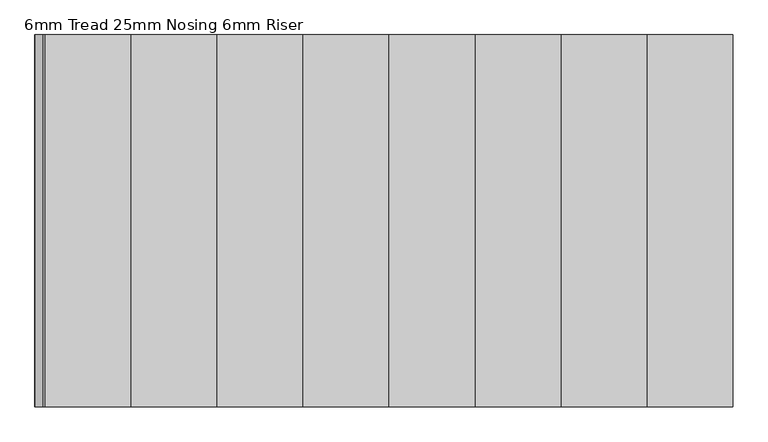
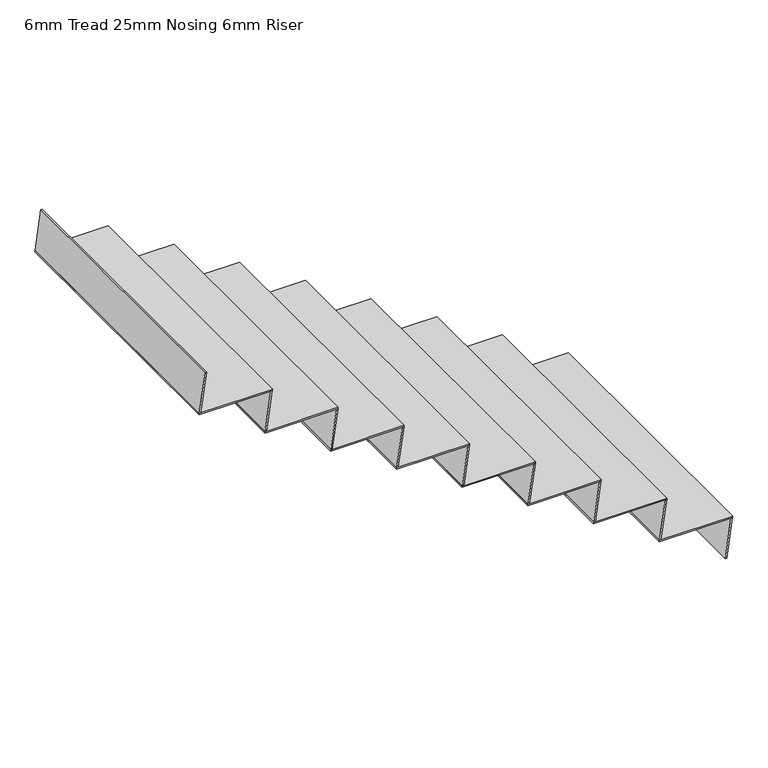
"""IFC4 building model written with IfcOpenShell, lengths in millimetres: stair flight geometry, 6mm Tread 25mm Nosing 6mm Riser."""

from ifc_helpers import new_model, si_unit, frame, origin, place, context, project, spatial, polyline, outline, extrude, source, transform, mapped, element, save


def stair_flight_6mm_tread_25mm_nosing_6mm_riser_aabb701a(model_context):
    return source(origin(), model_context, "Body", "SweptSolid", [
        extrude(outline(polyline([(18588.2352941, 16350.0), (18588.2352941, 16043.9400908), (18582.2352941, 16043.0900908), (18582.2352941, 16349.15), (18588.2352941, 16350.0)])), frame((0.0, 12030.4345331, 0.0), z_axis=(0.0, 1.0, 0.0), x_axis=(0.0, 0.0, 1.0)), (0.0, 0.0, 1.0), 1190.0),
        extrude(outline(polyline([(18582.2352941, 16349.15), (18582.2352941, 16343.0900908), (18411.7647059, 16318.9400908), (18411.7647059, 16325.0), (18582.2352941, 16349.15)])), frame((0.0, 12030.4345331, 0.0), z_axis=(0.0, 1.0, 0.0), x_axis=(0.0, 0.0, 1.0)), (0.0, 0.0, 1.0), 1190.0),
        extrude(outline(polyline([(18758.7058824, 16074.15), (18758.7058824, 16068.0900908), (18588.2352941, 16043.9400908), (18588.2352941, 16050.0), (18758.7058824, 16074.15)])), frame((0.0, 12030.4345331, 0.0), z_axis=(0.0, 1.0, 0.0), x_axis=(0.0, 0.0, 1.0)), (0.0, 0.0, 1.0), 1190.0),
        extrude(outline(polyline([(18764.7058824, 16075.0), (18764.7058824, 15768.9400908), (18758.7058824, 15768.0900908), (18758.7058824, 16074.15), (18764.7058824, 16075.0)])), frame((0.0, 12030.4345331, 0.0), z_axis=(0.0, 1.0, 0.0), x_axis=(0.0, 0.0, 1.0)), (0.0, 0.0, 1.0), 1190.0),
        extrude(outline(polyline([(18935.1764706, 15799.15), (18935.1764706, 15793.0900908), (18764.7058824, 15768.9400908), (18764.7058824, 15775.0), (18935.1764706, 15799.15)])), frame((0.0, 12030.4345331, 0.0), z_axis=(0.0, 1.0, 0.0), x_axis=(0.0, 0.0, 1.0)), (0.0, 0.0, 1.0), 1190.0),
        extrude(outline(polyline([(18941.1764706, 15800.0), (18941.1764706, 15493.9400908), (18935.1764706, 15493.0900908), (18935.1764706, 15799.15), (18941.1764706, 15800.0)])), frame((0.0, 12030.4345331, 0.0), z_axis=(0.0, 1.0, 0.0), x_axis=(0.0, 0.0, 1.0)), (0.0, 0.0, 1.0), 1190.0),
        extrude(outline(polyline([(19111.6470588, 15524.15), (19111.6470588, 15518.0900908), (18941.1764706, 15493.9400908), (18941.1764706, 15500.0), (19111.6470588, 15524.15)])), frame((0.0, 12030.4345331, 0.0), z_axis=(0.0, 1.0, 0.0), x_axis=(0.0, 0.0, 1.0)), (0.0, 0.0, 1.0), 1190.0),
        extrude(outline(polyline([(19117.6470588, 15525.0), (19117.6470588, 15218.9400908), (19111.6470588, 15218.0900908), (19111.6470588, 15524.15), (19117.6470588, 15525.0)])), frame((0.0, 12030.4345331, 0.0), z_axis=(0.0, 1.0, 0.0), x_axis=(0.0, 0.0, 1.0)), (0.0, 0.0, 1.0), 1190.0),
        extrude(outline(polyline([(19288.1176471, 15249.15), (19288.1176471, 15243.0900908), (19117.6470588, 15218.9400908), (19117.6470588, 15225.0), (19288.1176471, 15249.15)])), frame((0.0, 12030.4345331, 0.0), z_axis=(0.0, 1.0, 0.0), x_axis=(0.0, 0.0, 1.0)), (0.0, 0.0, 1.0), 1190.0),
        extrude(outline(polyline([(19294.1176471, 15250.0), (19294.1176471, 14943.9400908), (19288.1176471, 14943.0900908), (19288.1176471, 15249.15), (19294.1176471, 15250.0)])), frame((0.0, 12030.4345331, 0.0), z_axis=(0.0, 1.0, 0.0), x_axis=(0.0, 0.0, 1.0)), (0.0, 0.0, 1.0), 1190.0),
        extrude(outline(polyline([(19464.5882353, 14974.15), (19464.5882353, 14968.0900908), (19294.1176471, 14943.9400908), (19294.1176471, 14950.0), (19464.5882353, 14974.15)])), frame((0.0, 12030.4345331, 0.0), z_axis=(0.0, 1.0, 0.0), x_axis=(0.0, 0.0, 1.0)), (0.0, 0.0, 1.0), 1190.0),
        extrude(outline(polyline([(19470.5882353, 14975.0), (19470.5882353, 14668.9400908), (19464.5882353, 14668.0900908), (19464.5882353, 14974.15), (19470.5882353, 14975.0)])), frame((0.0, 12030.4345331, 0.0), z_axis=(0.0, 1.0, 0.0), x_axis=(0.0, 0.0, 1.0)), (0.0, 0.0, 1.0), 1190.0),
        extrude(outline(polyline([(19641.0588235, 14699.15), (19641.0588235, 14693.0900908), (19470.5882353, 14668.9400908), (19470.5882353, 14675.0), (19641.0588235, 14699.15)])), frame((0.0, 12030.4345331, 0.0), z_axis=(0.0, 1.0, 0.0), x_axis=(0.0, 0.0, 1.0)), (0.0, 0.0, 1.0), 1190.0),
        extrude(outline(polyline([(19647.0588235, 14700.0), (19647.0588235, 14393.9400908), (19641.0588235, 14393.0900908), (19641.0588235, 14699.15), (19647.0588235, 14700.0)])), frame((0.0, 12030.4345331, 0.0), z_axis=(0.0, 1.0, 0.0), x_axis=(0.0, 0.0, 1.0)), (0.0, 0.0, 1.0), 1190.0),
        extrude(outline(polyline([(19817.5294118, 14424.15), (19817.5294118, 14418.0900908), (19647.0588235, 14393.9400908), (19647.0588235, 14400.0), (19817.5294118, 14424.15)])), frame((0.0, 12030.4345331, 0.0), z_axis=(0.0, 1.0, 0.0), x_axis=(0.0, 0.0, 1.0)), (0.0, 0.0, 1.0), 1190.0),
        extrude(outline(polyline([(19994.0, 14149.15), (19994.0, 14143.0900908), (19823.5294118, 14118.9400908), (19823.5294118, 14125.0), (19994.0, 14149.15)])), frame((0.0, 12030.4345331, 0.0), z_axis=(0.0, 1.0, 0.0), x_axis=(0.0, 0.0, 1.0)), (0.0, 0.0, 1.0), 1190.0),
        extrude(outline(polyline([(19823.5294118, 14425.0), (19823.5294118, 14118.9400908), (19817.5294118, 14118.0900908), (19817.5294118, 14424.15), (19823.5294118, 14425.0)])), frame((0.0, 12030.4345331, 0.0), z_axis=(0.0, 1.0, 0.0), x_axis=(0.0, 0.0, 1.0)), (0.0, 0.0, 1.0), 1190.0),
    ])


if __name__ == "__main__":
    model = new_model("IFC4")
    model_context = context("Model", 3, world=origin())
    ifc_project = project(units=[si_unit("LENGTHUNIT", "METRE", prefix="MILLI")], contexts=[model_context])
    site = spatial("IfcSite", under=ifc_project)
    building = spatial("IfcBuilding", under=site)
    placement = place(None, origin())
    stair_flight_6mm_tread_25mm_nosing_6mm_riser_shape = stair_flight_6mm_tread_25mm_nosing_6mm_riser_aabb701a(model_context)
    element("IfcStairFlight", 1, ObjectType="6mm Tread 25mm Nosing 6mm Riser", at=placement, inside=building, context=model_context, shape_type="MappedRepresentation", body=[
        mapped(stair_flight_6mm_tread_25mm_nosing_6mm_riser_shape, transform((0.0, 0.0, 0.0), x_axis=(1.0, 0.0, 0.0), y_axis=(0.0, 1.0, 0.0), z_axis=(0.0, 0.0, 1.0))),
    ])
    save(model, "model.ifc")

# Revit data of these elements
# Element 1 (IfcStairFlight, "6mm Tread 25mm Nosing 6mm Riser")
#   Materials on its faces: "Steel, Paint Finish, Dark Gray"
# Materials
#   "Steel, Paint Finish, Dark Gray": class "Metal", colour RGB 89 89 89, transparency 0, Description = "Steel, paint finish, dark gray, glossy", Cost = 0
